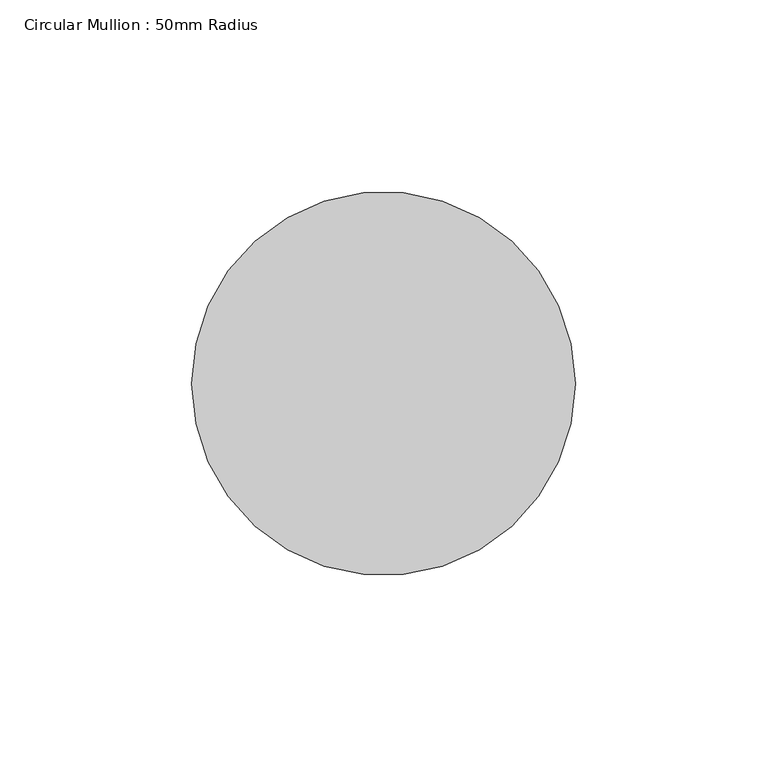
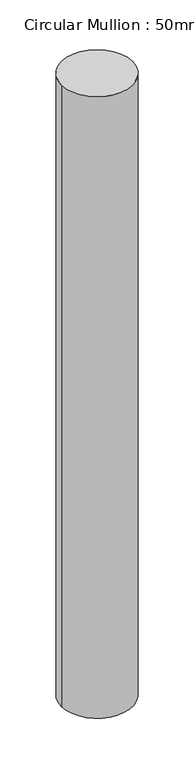
"""IFC4 building model written with IfcOpenShell, lengths in millimetres: member geometry, Circular Mullion : 50mm Radius."""

import ifcopenshell
import ifcopenshell.guid

model = None  # the IFC model being written
_history = None  # IfcOwnerHistory: only IFC2X3 demands one
_inside = {}  # id of a spatial element -> (the spatial element, [elements in it])
_under = {}  # id of a project, library or spatial element -> (it, [spatial elements below it])
_declared = {}  # id of a project -> (the project, [libraries it declares])
_typed = {}  # id of a type object -> (the type object, [elements of that type])
_made_of = {}  # id of a material, layer set ... -> (it, [elements and type objects made of it])


def new_model(schema):
    """Start an empty IFC model of exactly this schema.

    Asked for "IFC4X3", IfcOpenShell would pick the latest addendum, in which some entities
    have other attributes; the version numbers below select the first issue.
    IFC2X3 requires an IfcOwnerHistory on every rooted entity: one is made here for all.
    """
    global model, _history
    if schema == "IFC4X3":
        model = ifcopenshell.file(schema_version=(4, 3, 0, 0))
    else:
        model = ifcopenshell.file(schema=schema)
    _inside.clear()
    _under.clear()
    _declared.clear()
    _typed.clear()
    _made_of.clear()
    _history = None
    if model.schema == "IFC2X3":
        org = make("IfcOrganization", Name="unknown")
        user = make(
            "IfcPersonAndOrganization",
            ThePerson=make("IfcPerson", FamilyName="unknown"),
            TheOrganization=org,
        )
        app = make(
            "IfcApplication",
            ApplicationDeveloper=org,
            Version="unknown",
            ApplicationFullName="unknown",
            ApplicationIdentifier="unknown",
        )
        _history = make(
            "IfcOwnerHistory",
            OwningUser=user,
            OwningApplication=app,
            ChangeAction="ADDED",
            CreationDate=0,
        )
    return model


def make(cls, **values):
    """One entity of the class cls with the attributes given. An attribute that is None is left unset."""
    return model.create_entity(
        cls, **{name: value for name, value in values.items() if value is not None}
    )


def rooted(cls, **values):
    """An entity with a GlobalId (a new one), such as an element, a storey or a relation."""
    return make(cls, GlobalId=ifcopenshell.guid.new(), OwnerHistory=_history, **values)


def si_unit(unit_type, name, prefix=None):
    """IfcSIUnit, for example si_unit("LENGTHUNIT", "METRE", prefix="MILLI")."""
    return make("IfcSIUnit", UnitType=unit_type, Prefix=prefix, Name=name)


def assignment(units):
    """IfcUnitAssignment: the units of a project."""
    return None if units is None else make("IfcUnitAssignment", Units=units)


def point(xyz):
    """IfcCartesianPoint."""
    return None if xyz is None else make("IfcCartesianPoint", Coordinates=xyz)


def direction(xyz):
    """IfcDirection."""
    return None if xyz is None else make("IfcDirection", DirectionRatios=xyz)


def frame(location, z_axis=None, x_axis=None):
    """IfcAxis2Placement3D, a coordinate frame: its origin and axes. An axis left out is left unset."""
    return make(
        "IfcAxis2Placement3D",
        Location=point(location),
        Axis=direction(z_axis),
        RefDirection=direction(x_axis),
    )


def frame_2d(location, x_axis=None):
    """IfcAxis2Placement2D, a coordinate frame in the plane: its origin and x axis."""
    return make(
        "IfcAxis2Placement2D", Location=point(location), RefDirection=direction(x_axis)
    )


def origin():
    """The frame at (0, 0, 0) with its axes left unset."""
    return frame((0.0, 0.0, 0.0))


def origin_2d():
    """The frame at (0, 0) in the plane with its x axis left unset."""
    return frame_2d((0.0, 0.0))


def place(relative_to, where):
    """IfcLocalPlacement: puts the frame where relative to a parent placement (None: the world)."""
    return make(
        "IfcLocalPlacement", PlacementRelTo=relative_to, RelativePlacement=where
    )


def context(
    kind, dimensions, precision=None, world=None, true_north=None, identifier=None
):
    """IfcGeometricRepresentationContext, for example the 3D "Model" context."""
    return make(
        "IfcGeometricRepresentationContext",
        ContextIdentifier=identifier,
        ContextType=kind,
        CoordinateSpaceDimension=dimensions,
        Precision=precision,
        WorldCoordinateSystem=world,
        TrueNorth=true_north,
    )


def project(units=None, contexts=None):
    """IfcProject with its units and contexts."""
    return rooted(
        "IfcProject",
        Name="project",
        RepresentationContexts=contexts,
        UnitsInContext=assignment(units),
    )


def spatial(cls, under=None, at=None, **own):
    """A site, building, storey or space (cls), placed at a placement, below another one or the project."""
    s = rooted(cls, ObjectPlacement=at, **own)
    if under is not None:
        _under.setdefault(under.id(), (under, []))[1].append(s)
    return s


def circle_curve(where, radius):
    """IfcCircle in the frame where."""
    return make("IfcCircle", Position=where, Radius=radius)


def trimmed(basis, trim1, trim2, sense, master):
    """IfcTrimmedCurve: the piece of a basis curve between two trims."""
    return make(
        "IfcTrimmedCurve",
        BasisCurve=basis,
        Trim1=trim1,
        Trim2=trim2,
        SenseAgreement=sense,
        MasterRepresentation=master,
    )


def segment(curve, same_sense, transition):
    """IfcCompositeCurveSegment."""
    return make(
        "IfcCompositeCurveSegment",
        Transition=transition,
        SameSense=same_sense,
        ParentCurve=curve,
    )


def composite_curve(segments, self_intersect=None):
    """IfcCompositeCurve: segments joined end to end."""
    return make("IfcCompositeCurve", Segments=segments, SelfIntersect=self_intersect)


def outline(outer, holes=None, kind="AREA"):
    """IfcArbitraryClosedProfileDef: a profile drawn as a closed curve; with holes, ...WithVoids."""
    if holes is None:
        return make("IfcArbitraryClosedProfileDef", ProfileType=kind, OuterCurve=outer)
    return make(
        "IfcArbitraryProfileDefWithVoids",
        ProfileType=kind,
        OuterCurve=outer,
        InnerCurves=holes,
    )


def extrude(swept, where, along, depth):
    """IfcExtrudedAreaSolid: the profile swept, set in the frame where, extruded along a direction by depth."""
    return make(
        "IfcExtrudedAreaSolid",
        SweptArea=swept,
        Position=where,
        ExtrudedDirection=direction(along),
        Depth=depth,
    )


def shape(context_of_items, identifier, shape_type, items):
    """IfcShapeRepresentation: the items that make up one representation, for example the "Body"."""
    return make(
        "IfcShapeRepresentation",
        ContextOfItems=context_of_items,
        RepresentationIdentifier=identifier,
        RepresentationType=shape_type,
        Items=items,
    )


def source(mapping_origin, context_of_items, identifier, shape_type, items):
    """IfcRepresentationMap: a shape defined once, which mapped items show again and again."""
    return make(
        "IfcRepresentationMap",
        MappingOrigin=mapping_origin,
        MappedRepresentation=shape(context_of_items, identifier, shape_type, items),
    )


def transform(
    local_origin,
    x_axis=None,
    y_axis=None,
    z_axis=None,
    scale=None,
    scale2=None,
    scale3=None,
    uniform=True,
):
    """IfcCartesianTransformationOperator3D, or its non-uniform kind. x_axis, y_axis, z_axis: its Axis1, 2, 3."""
    if uniform:
        return make(
            "IfcCartesianTransformationOperator3D",
            Axis1=direction(x_axis),
            Axis2=direction(y_axis),
            LocalOrigin=point(local_origin),
            Scale=scale,
            Axis3=direction(z_axis),
        )
    return make(
        "IfcCartesianTransformationOperator3DnonUniform",
        Axis1=direction(x_axis),
        Axis2=direction(y_axis),
        LocalOrigin=point(local_origin),
        Scale=scale,
        Axis3=direction(z_axis),
        Scale2=scale2,
        Scale3=scale3,
    )


def mapped(mapping_source, mapping_target):
    """IfcMappedItem: shows the shape of a source again, moved by a transform."""
    return make(
        "IfcMappedItem", MappingSource=mapping_source, MappingTarget=mapping_target
    )


def made_of(thing, what):
    """Note that an element or type object is made of a material, layer set ...; save() writes the relation."""
    if what is not None:
        _made_of.setdefault(what.id(), (what, []))[1].append(thing)
    return thing


def element(
    cls,
    number,
    at=None,
    inside=None,
    cuts=None,
    type_object=None,
    material=None,
    context=None,
    identifier="Body",
    shape_type=None,
    held_by="IfcProductDefinitionShape",
    body=None,
    shapes=None,
    **own,
):
    """One element of the class cls, such as IfcWall. Its Tag is "e" and its number.

    at: its placement. inside: the storey or other place that contains it. cuts: it is an
    opening in that element (IfcRelVoidsElement). A single representation is given by context,
    identifier, shape_type and body (its items); several are given by shapes. held_by: the class
    of the entity that holds the representations. save() writes the other relations.
    """
    e = rooted(cls, Tag="e%d" % number, ObjectPlacement=at, **own)
    if body is not None:
        shapes = [shape(context, identifier, shape_type, body)]
    if shapes is not None:
        e.Representation = make(held_by, Representations=shapes)
    if inside is not None:
        _inside.setdefault(inside.id(), (inside, []))[1].append(e)
    if cuts is not None:
        rooted(
            "IfcRelVoidsElement", RelatingBuildingElement=cuts, RelatedOpeningElement=e
        )
    if type_object is not None:
        _typed.setdefault(type_object.id(), (type_object, []))[1].append(e)
    return made_of(e, material)


def aggregate(whole, parts):
    """IfcRelAggregates: a whole, such as a stair, and the parts it consists of."""
    return rooted("IfcRelAggregates", RelatingObject=whole, RelatedObjects=parts)


def save(model, path):
    """Write the relations noted so far, then the file.

    IfcRelAggregates (storeys below a building ...), IfcRelContainedInSpatialStructure (elements
    in a storey), IfcRelDefinesByType, IfcRelAssociatesMaterial and IfcRelDeclares: one each for
    every whole, place, type object, material and project.
    """
    for whole, parts in _under.values():
        aggregate(whole, parts)
    for where, things in _inside.values():
        rooted(
            "IfcRelContainedInSpatialStructure",
            RelatedElements=things,
            RelatingStructure=where,
        )
    for kind, things in _typed.values():
        rooted("IfcRelDefinesByType", RelatedObjects=things, RelatingType=kind)
    for what, things in _made_of.values():
        rooted("IfcRelAssociatesMaterial", RelatedObjects=things, RelatingMaterial=what)
    for by, libraries in _declared.values():
        rooted("IfcRelDeclares", RelatingContext=by, RelatedDefinitions=libraries)
    model.write(path)


def circular_mullion_50mm_radius_3b5781b3(model_context):
    return source(origin(), model_context, "Body", "SweptSolid", [
        extrude(outline(composite_curve([segment(trimmed(circle_curve(origin_2d(), 50.0), [point((50.0, 0.0))], [point((-50.0, 0.0))], False, "CARTESIAN"), True, "CONTINUOUS"), segment(trimmed(circle_curve(origin_2d(), 50.0), [point((-50.0, 0.0))], [point((50.0, 0.0))], False, "CARTESIAN"), True, "CONTINUOUS")], self_intersect=False)), frame((0.0, 0.0, -923.7327329), z_axis=(0.0, 0.0, 1.0), x_axis=(1.0, 0.0, 0.0)), (0.0, 0.0, 1.0), 923.7327329),
    ])


if __name__ == "__main__":
    model = new_model("IFC4")
    model_context = context("Model", 3, world=origin())
    ifc_project = project(units=[si_unit("LENGTHUNIT", "METRE", prefix="MILLI")], contexts=[model_context])
    site = spatial("IfcSite", under=ifc_project)
    building = spatial("IfcBuilding", under=site)
    placement = place(None, origin())
    circular_mullion_50mm_radius_shape = circular_mullion_50mm_radius_3b5781b3(model_context)
    element("IfcMember", 1, ObjectType="Circular Mullion : 50mm Radius", at=placement, inside=building, context=model_context, shape_type="MappedRepresentation", body=[
        mapped(circular_mullion_50mm_radius_shape, transform((0.0, 0.0, 0.0), x_axis=(1.0, 0.0, 0.0), y_axis=(0.0, 1.0, 0.0), z_axis=(0.0, 0.0, 1.0))),
    ])
    save(model, "model.ifc")

# Revit data of these elements
# Type "Circular Mullion : 50mm Radius"
#   built-in parameter 1007350 = 0.164042 (stored number, unit not read)
# Element 1 (IfcMember, "Circular Mullion : 50mm Radius")
#   Materials on its faces: "Aluminium"
# Materials
#   "Aluminium": class "Metal", colour RGB 247 247 247, transparency 0, Description = "Aluminium 6061", Cost = 0
